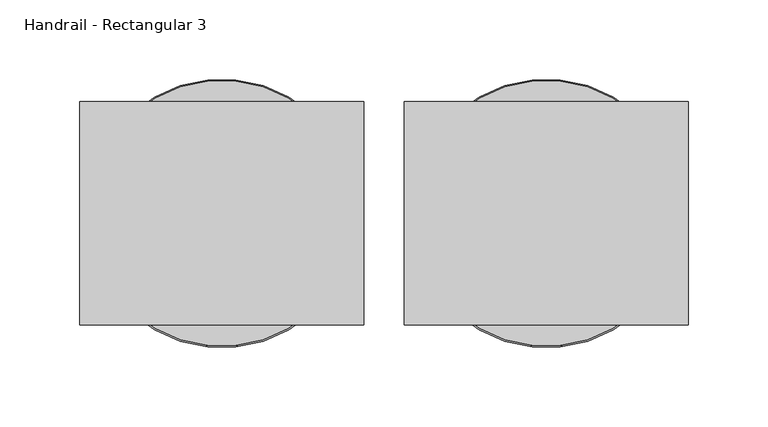
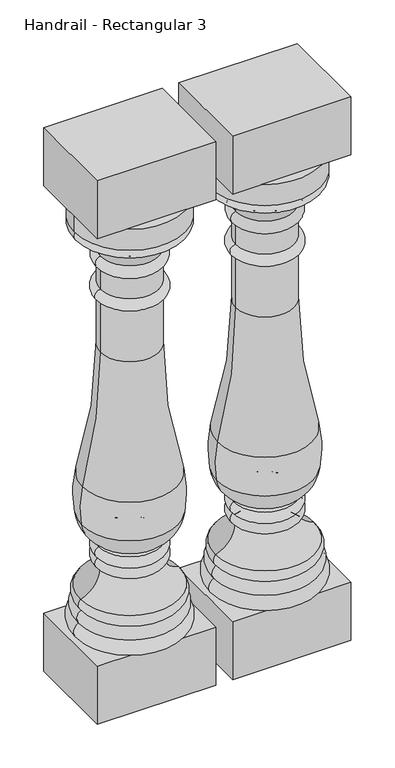
"""IFC4 building model written with IfcOpenShell, lengths in millimetres: railing geometry, Handrail - Rectangular 3."""

from ifc_helpers import new_model, si_unit, point, frame, origin, place, context, project, spatial, polyline, circle_curve, ellipse_curve, trimmed, outline, extrude, source, transform, mapped, element, save
from ifc_brep_helpers import plane_surface, cylinder_surface, revolved_surface, advanced_brep


def handrail_rectangular_3_94038515(model_context):
    return source(origin(), model_context, "Body", "SolidModel", [
        advanced_brep(
        [(12017.1084395, -1665.6164768, 849.3125), (12183.7959395, -1665.6164768, 849.3125), (12183.7959395, -1665.6164768, 882.65), (12017.1084395, -1665.6164768, 882.65), (12020.2834395, -1665.6164768, 849.3125), (12180.6209395, -1665.6164768, 849.3125), (12020.2834395, -1665.6164768, 835.025), (12180.6209395, -1665.6164768, 835.025), (12056.7959395, -1665.6164768, 796.925), (12144.1084395, -1665.6164768, 796.925), (12056.7959395, -1665.6164768, 777.875), (12144.1084395, -1665.6164768, 777.875), (12056.7959395, -1665.6164768, 744.5375), (12144.1084395, -1665.6164768, 744.5375), (12056.7959395, -1665.6164768, 727.075), (12144.1084395, -1665.6164768, 727.075), (12056.7959395, -1665.6164768, 644.525), (12144.1084395, -1665.6164768, 644.525), (12029.6074221, -1665.6164768, 440.2065586), (12171.296957, -1665.6164768, 440.2065586), (12028.4170661, -1665.6164768, 379.6643134), (12172.487313, -1665.6164768, 379.6643134), (12055.6281246, -1665.6164768, 340.8286685), (12145.2762545, -1665.6164768, 340.8286685), (12053.9028429, -1665.6164768, 336.3463085), (12147.0015362, -1665.6164768, 336.3463085), (12052.8271895, -1665.6164768, 319.0875), (12148.0771895, -1665.6164768, 319.0875), (12056.0021895, -1665.6164768, 301.625), (12144.9021895, -1665.6164768, 301.625), (12026.6334395, -1665.6164768, 261.9375), (12174.2709395, -1665.6164768, 261.9375), (12027.4271895, -1665.6164768, 244.475), (12173.4771895, -1665.6164768, 244.475), (12023.4584395, -1665.6164768, 225.425), (12177.4459395, -1665.6164768, 225.425), (12020.2834395, -1665.6164768, 203.2), (12180.6209395, -1665.6164768, 203.2), (12100.4521895, -1665.6164768, 203.2), (12100.4521895, -1665.6164768, 882.65)],
        [
            (0, 1, circle_curve(frame((12100.4521895, -1665.6164768, 849.3125), z_axis=(0.0, 0.0, 1.0), x_axis=(1.0, 0.0, 0.0)), 83.34375)),
            (1, 2),
            (2, 3, circle_curve(frame((12100.4521895, -1665.6164768, 882.65), z_axis=(0.0, 0.0, -1.0), x_axis=(1.0, 0.0, 0.0)), 83.34375)),
            (3, 0),
            (1, 0, circle_curve(frame((12100.4521895, -1665.6164768, 849.3125), z_axis=(0.0, 0.0, 1.0), x_axis=(1.0, 0.0, 0.0)), 83.34375)),
            (3, 2, circle_curve(frame((12100.4521895, -1665.6164768, 882.65), z_axis=(0.0, 0.0, -1.0), x_axis=(1.0, 0.0, 0.0)), 83.34375)),
            (4, 5, circle_curve(frame((12100.4521895, -1665.6164768, 849.3125), z_axis=(0.0, 0.0, 1.0), x_axis=(1.0, 0.0, 0.0)), 80.16875)),
            (5, 1),
            (0, 4),
            (5, 4, circle_curve(frame((12100.4521895, -1665.6164768, 849.3125), z_axis=(0.0, 0.0, 1.0), x_axis=(1.0, 0.0, 0.0)), 80.16875)),
            (6, 7, circle_curve(frame((12100.4521895, -1665.6164768, 835.025), z_axis=(0.0, 0.0, 1.0), x_axis=(1.0, 0.0, 0.0)), 80.16875)),
            (7, 5, circle_curve(frame((12174.1717208, -1665.6164768, 842.16875), z_axis=(0.0, -1.0, 0.0), x_axis=(1.0, 0.0, 0.0)), 9.6242187)),
            (4, 6, circle_curve(frame((12026.7326583, -1665.6164768, 842.16875), z_axis=(0.0, -1.0, 0.0), x_axis=(-1.0, 0.0, 0.0)), 9.6242187)),
            (7, 6, circle_curve(frame((12100.4521895, -1665.6164768, 835.025), z_axis=(0.0, 0.0, 1.0), x_axis=(1.0, 0.0, 0.0)), 80.16875)),
            (8, 9, circle_curve(frame((12100.4521895, -1665.6164768, 796.925), z_axis=(0.0, 0.0, 1.0), x_axis=(1.0, 0.0, 0.0)), 43.65625)),
            (9, 7, circle_curve(frame((12199.525244, -1665.6164768, 780.362802), z_axis=(0.0, 1.0, 0.0), x_axis=(1.0, 0.0, 0.0)), 57.8388159)),
            (6, 8, circle_curve(frame((12001.3791351, -1665.6164768, 780.362802), z_axis=(0.0, 1.0, 0.0), x_axis=(-1.0, 0.0, 0.0)), 57.8388159)),
            (9, 8, circle_curve(frame((12100.4521895, -1665.6164768, 796.925), z_axis=(0.0, 0.0, 1.0), x_axis=(1.0, 0.0, 0.0)), 43.65625)),
            (10, 11, circle_curve(frame((12100.4521895, -1665.6164768, 777.875), z_axis=(0.0, 0.0, 1.0), x_axis=(1.0, 0.0, 0.0)), 43.65625)),
            (11, 9, circle_curve(frame((12142.3621895, -1665.6164768, 787.4), z_axis=(0.0, -1.0, 0.0), x_axis=(1.0, 0.0, 0.0)), 9.68375)),
            (8, 10, circle_curve(frame((12058.5421895, -1665.6164768, 787.4), z_axis=(0.0, -1.0, 0.0), x_axis=(-1.0, 0.0, 0.0)), 9.68375)),
            (11, 10, circle_curve(frame((12100.4521895, -1665.6164768, 777.875), z_axis=(0.0, 0.0, 1.0), x_axis=(1.0, 0.0, 0.0)), 43.65625)),
            (12, 13, circle_curve(frame((12100.4521895, -1665.6164768, 744.5375), z_axis=(0.0, 0.0, 1.0), x_axis=(1.0, 0.0, 0.0)), 43.65625)),
            (13, 11),
            (10, 12),
            (13, 12, circle_curve(frame((12100.4521895, -1665.6164768, 744.5375), z_axis=(0.0, 0.0, 1.0), x_axis=(1.0, 0.0, 0.0)), 43.65625)),
            (14, 15, circle_curve(frame((12100.4521895, -1665.6164768, 727.075), z_axis=(0.0, 0.0, 1.0), x_axis=(1.0, 0.0, 0.0)), 43.65625)),
            (15, 13, circle_curve(frame((12144.1084395, -1665.6164768, 735.80625), z_axis=(0.0, -1.0, 0.0), x_axis=(1.0, 0.0, 0.0)), 8.73125)),
            (12, 14, circle_curve(frame((12056.7959395, -1665.6164768, 735.80625), z_axis=(0.0, -1.0, 0.0), x_axis=(-1.0, 0.0, 0.0)), 8.73125)),
            (15, 14, circle_curve(frame((12100.4521895, -1665.6164768, 727.075), z_axis=(0.0, 0.0, 1.0), x_axis=(1.0, 0.0, 0.0)), 43.65625)),
            (16, 17, circle_curve(frame((12100.4521895, -1665.6164768, 644.525), z_axis=(0.0, 0.0, 1.0), x_axis=(1.0, 0.0, 0.0)), 43.65625)),
            (17, 15),
            (14, 16),
            (17, 16, circle_curve(frame((12100.4521895, -1665.6164768, 644.525), z_axis=(0.0, 0.0, 1.0), x_axis=(1.0, 0.0, 0.0)), 43.65625)),
            (18, 19, circle_curve(frame((12100.4521895, -1665.6164768, 440.2065586), z_axis=(0.0, 0.0, 1.0), x_axis=(1.0, 0.0, 0.0)), 70.8447675)),
            (19, 17, circle_curve(frame((12878.8851891, -1665.6164768, 638.333048), z_axis=(0.0, 1.0, 0.0), x_axis=(1.0, 0.0, 0.0)), 734.8028389)),
            (16, 18, circle_curve(frame((11322.01919, -1665.6164768, 638.333048), z_axis=(0.0, 1.0, 0.0), x_axis=(-1.0, 0.0, 0.0)), 734.8028389)),
            (19, 18, circle_curve(frame((12100.4521895, -1665.6164768, 440.2065586), z_axis=(0.0, 0.0, 1.0), x_axis=(1.0, 0.0, 0.0)), 70.8447675)),
            (20, 21, circle_curve(frame((12100.4521895, -1665.6164768, 379.6643134), z_axis=(0.0, 0.0, 1.0), x_axis=(1.0, 0.0, 0.0)), 72.0351235)),
            (21, 19, circle_curve(frame((12013.3983349, -1665.6164768, 406.819198), z_axis=(0.0, -1.0, 0.0), x_axis=(1.0, 0.0, 0.0)), 161.3898718)),
            (18, 20, circle_curve(frame((12187.5060442, -1665.6164768, 406.819198), z_axis=(0.0, -1.0, 0.0), x_axis=(-1.0, 0.0, 0.0)), 161.3898718)),
            (21, 20, circle_curve(frame((12100.4521895, -1665.6164768, 379.6643134), z_axis=(0.0, 0.0, 1.0), x_axis=(1.0, 0.0, 0.0)), 72.0351235)),
            (22, 23, circle_curve(frame((12100.4521895, -1665.6164768, 340.8286685), z_axis=(0.0, 0.0, 1.0), x_axis=(1.0, 0.0, 0.0)), 44.8240649)),
            (23, 21, circle_curve(frame((12122.7572912, -1665.6164768, 385.5579203), z_axis=(0.0, -1.0, 0.0), x_axis=(1.0, 0.0, 0.0)), 50.0780358)),
            (20, 22, circle_curve(frame((12078.1470879, -1665.6164768, 385.5579203), z_axis=(0.0, -1.0, 0.0), x_axis=(-1.0, 0.0, 0.0)), 50.0780358)),
            (23, 22, circle_curve(frame((12100.4521895, -1665.6164768, 340.8286685), z_axis=(0.0, 0.0, 1.0), x_axis=(1.0, 0.0, 0.0)), 44.8240649)),
            (24, 25, circle_curve(frame((12100.4521895, -1665.6164768, 336.3463085), z_axis=(0.0, 0.0, 1.0), x_axis=(1.0, 0.0, 0.0)), 46.5493467)),
            (25, 23, circle_curve(frame((12148.0771895, -1665.6164768, 339.3335472), z_axis=(0.0, 1.0, 0.0), x_axis=(1.0, 0.0, 0.0)), 3.175)),
            (22, 24, circle_curve(frame((12052.8271895, -1665.6164768, 339.3335472), z_axis=(0.0, 1.0, 0.0), x_axis=(-1.0, 0.0, 0.0)), 3.175)),
            (25, 24, circle_curve(frame((12100.4521895, -1665.6164768, 336.3463085), z_axis=(0.0, 0.0, 1.0), x_axis=(1.0, 0.0, 0.0)), 46.5493467)),
            (26, 27, circle_curve(frame((12100.4521895, -1665.6164768, 319.0875), z_axis=(0.0, 0.0, 1.0), x_axis=(1.0, 0.0, 0.0)), 47.625)),
            (27, 25, circle_curve(frame((12143.0008248, -1665.6164768, 327.4340404), z_axis=(0.0, -1.0, 0.0), x_axis=(1.0, 0.0, 0.0)), 9.7690437)),
            (24, 26, circle_curve(frame((12057.9035543, -1665.6164768, 327.4340404), z_axis=(0.0, -1.0, 0.0), x_axis=(-1.0, 0.0, 0.0)), 9.7690437)),
            (27, 26, circle_curve(frame((12100.4521895, -1665.6164768, 319.0875), z_axis=(0.0, 0.0, 1.0), x_axis=(1.0, 0.0, 0.0)), 47.625)),
            (28, 29, circle_curve(frame((12100.4521895, -1665.6164768, 301.625), z_axis=(0.0, 0.0, 1.0), x_axis=(1.0, 0.0, 0.0)), 44.45)),
            (29, 27, circle_curve(frame((12143.4635177, -1665.6164768, 310.9064631), z_axis=(0.0, -1.0, 0.0), x_axis=(1.0, 0.0, 0.0)), 9.3923018)),
            (26, 28, circle_curve(frame((12057.4408614, -1665.6164768, 310.9064631), z_axis=(0.0, -1.0, 0.0), x_axis=(-1.0, 0.0, 0.0)), 9.3923018)),
            (29, 28, circle_curve(frame((12100.4521895, -1665.6164768, 301.625), z_axis=(0.0, 0.0, 1.0), x_axis=(1.0, 0.0, 0.0)), 44.45)),
            (30, 31, circle_curve(frame((12100.4521895, -1665.6164768, 261.9375), z_axis=(0.0, 0.0, 1.0), x_axis=(1.0, 0.0, 0.0)), 73.81875)),
            (31, 29, circle_curve(frame((12186.4024429, -1665.6164768, 301.625), z_axis=(0.0, 1.0, 0.0), x_axis=(1.0, 0.0, 0.0)), 41.5002534)),
            (28, 30, circle_curve(frame((12014.5019362, -1665.6164768, 301.625), z_axis=(0.0, 1.0, 0.0), x_axis=(-1.0, 0.0, 0.0)), 41.5002534)),
            (31, 30, circle_curve(frame((12100.4521895, -1665.6164768, 261.9375), z_axis=(0.0, 0.0, 1.0), x_axis=(1.0, 0.0, 0.0)), 73.81875)),
            (32, 33, circle_curve(frame((12100.4521895, -1665.6164768, 244.475), z_axis=(0.0, 0.0, 1.0), x_axis=(1.0, 0.0, 0.0)), 73.025)),
            (33, 31, circle_curve(frame((12164.9664257, -1665.6164768, 253.6111427), z_axis=(0.0, -1.0, 0.0), x_axis=(1.0, 0.0, 0.0)), 12.4860804)),
            (30, 32, circle_curve(frame((12035.9379534, -1665.6164768, 253.6111427), z_axis=(0.0, -1.0, 0.0), x_axis=(-1.0, 0.0, 0.0)), 12.4860804)),
            (33, 32, circle_curve(frame((12100.4521895, -1665.6164768, 244.475), z_axis=(0.0, 0.0, 1.0), x_axis=(1.0, 0.0, 0.0)), 73.025)),
            (34, 35, circle_curve(frame((12100.4521895, -1665.6164768, 225.425), z_axis=(0.0, 0.0, 1.0), x_axis=(1.0, 0.0, 0.0)), 76.99375)),
            (35, 33, circle_curve(frame((12166.8024736, -1665.6164768, 233.1460227), z_axis=(0.0, -1.0, 0.0), x_axis=(1.0, 0.0, 0.0)), 13.1490516)),
            (32, 34, circle_curve(frame((12034.1019054, -1665.6164768, 233.1460227), z_axis=(0.0, -1.0, 0.0), x_axis=(-1.0, 0.0, 0.0)), 13.1490516)),
            (35, 34, circle_curve(frame((12100.4521895, -1665.6164768, 225.425), z_axis=(0.0, 0.0, 1.0), x_axis=(1.0, 0.0, 0.0)), 76.99375)),
            (36, 37, circle_curve(frame((12100.4521895, -1665.6164768, 203.2), z_axis=(0.0, 0.0, 1.0), x_axis=(1.0, 0.0, 0.0)), 80.16875)),
            (37, 35, circle_curve(frame((12170.4722788, -1665.6164768, 213.089477), z_axis=(0.0, -1.0, 0.0), x_axis=(1.0, 0.0, 0.0)), 14.1702883)),
            (34, 36, circle_curve(frame((12030.4321003, -1665.6164768, 213.089477), z_axis=(0.0, -1.0, 0.0), x_axis=(-1.0, 0.0, 0.0)), 14.1702883)),
            (37, 36, circle_curve(frame((12100.4521895, -1665.6164768, 203.2), z_axis=(0.0, 0.0, 1.0), x_axis=(1.0, 0.0, 0.0)), 80.16875)),
            (38, 37),
            (36, 38),
            (2, 39),
            (39, 3),
        ],
        [
            cylinder_surface(frame((12100.4521895, -1665.6164768, 831.85), z_axis=(0.0, 0.0, -1.0), x_axis=(1.0, 0.0, 0.0)), 83.34375),
            plane_surface(frame((12100.4521895, -1665.6164768, 849.3125), z_axis=(0.0, 0.0, -1.0), x_axis=(1.0, 0.0, 0.0))),
            revolved_surface(trimmed(ellipse_curve(frame((12174.1717208, -1665.6164768, 842.16875), z_axis=(0.0, 1.0, 0.0), x_axis=(1.0, 0.0, 0.0)), 9.6242187, 9.6242187), [point((12180.6209395, -1665.6164768, 849.3125))], [point((12180.6209395, -1665.6164768, 835.025))], True, "CARTESIAN"), (12100.4521895, -1665.6164768, 831.85), (0.0, 0.0, -1.0)),
            revolved_surface(trimmed(ellipse_curve(frame((12199.525244, -1665.6164768, 780.362802), z_axis=(0.0, -1.0, 0.0), x_axis=(1.0, 0.0, 0.0)), 57.8388159, 57.8388159), [point((12180.6209395, -1665.6164768, 835.025))], [point((12144.1084395, -1665.6164768, 796.925))], True, "CARTESIAN"), (12100.4521895, -1665.6164768, 831.85), (0.0, 0.0, -1.0)),
            revolved_surface(trimmed(ellipse_curve(frame((12142.3621895, -1665.6164768, 787.4), z_axis=(0.0, 1.0, 0.0), x_axis=(1.0, 0.0, 0.0)), 9.68375, 9.68375), [point((12144.1084395, -1665.6164768, 796.925))], [point((12144.1084395, -1665.6164768, 777.875))], True, "CARTESIAN"), (12100.4521895, -1665.6164768, 831.85), (0.0, 0.0, -1.0)),
            cylinder_surface(frame((12100.4521895, -1665.6164768, 831.85), z_axis=(0.0, 0.0, -1.0), x_axis=(1.0, 0.0, 0.0)), 43.65625),
            revolved_surface(trimmed(ellipse_curve(frame((12144.1084395, -1665.6164768, 735.80625), z_axis=(0.0, 1.0, 0.0), x_axis=(1.0, 0.0, 0.0)), 8.73125, 8.73125), [point((12144.1084395, -1665.6164768, 744.5375))], [point((12144.1084395, -1665.6164768, 727.075))], True, "CARTESIAN"), (12100.4521895, -1665.6164768, 831.85), (0.0, 0.0, -1.0)),
            revolved_surface(trimmed(ellipse_curve(frame((12878.8851891, -1665.6164768, 638.333048), z_axis=(0.0, -1.0, 0.0), x_axis=(1.0, 0.0, 0.0)), 734.8028389, 734.8028389), [point((12144.1084395, -1665.6164768, 644.525))], [point((12171.296957, -1665.6164768, 440.2065586))], True, "CARTESIAN"), (12100.4521895, -1665.6164768, 831.85), (0.0, 0.0, -1.0)),
            revolved_surface(trimmed(ellipse_curve(frame((12013.3983349, -1665.6164768, 406.819198), z_axis=(0.0, 1.0, 0.0), x_axis=(1.0, 0.0, 0.0)), 161.3898718, 161.3898718), [point((12171.296957, -1665.6164768, 440.2065586))], [point((12172.487313, -1665.6164768, 379.6643134))], True, "CARTESIAN"), (12100.4521895, -1665.6164768, 831.85), (0.0, 0.0, -1.0)),
            revolved_surface(trimmed(ellipse_curve(frame((12122.7572912, -1665.6164768, 385.5579203), z_axis=(0.0, 1.0, 0.0), x_axis=(1.0, 0.0, 0.0)), 50.0780358, 50.0780358), [point((12172.487313, -1665.6164768, 379.6643134))], [point((12145.2762545, -1665.6164768, 340.8286685))], True, "CARTESIAN"), (12100.4521895, -1665.6164768, 831.85), (0.0, 0.0, -1.0)),
            revolved_surface(trimmed(ellipse_curve(frame((12148.0771895, -1665.6164768, 339.3335472), z_axis=(0.0, -1.0, 0.0), x_axis=(1.0, 0.0, 0.0)), 3.175, 3.175), [point((12145.2762545, -1665.6164768, 340.8286685))], [point((12147.0015362, -1665.6164768, 336.3463085))], True, "CARTESIAN"), (12100.4521895, -1665.6164768, 831.85), (0.0, 0.0, -1.0)),
            revolved_surface(trimmed(ellipse_curve(frame((12143.0008248, -1665.6164768, 327.4340404), z_axis=(0.0, 1.0, 0.0), x_axis=(1.0, 0.0, 0.0)), 9.7690437, 9.7690437), [point((12147.0015362, -1665.6164768, 336.3463085))], [point((12148.0771895, -1665.6164768, 319.0875))], True, "CARTESIAN"), (12100.4521895, -1665.6164768, 831.85), (0.0, 0.0, -1.0)),
            revolved_surface(trimmed(ellipse_curve(frame((12143.4635177, -1665.6164768, 310.9064631), z_axis=(0.0, 1.0, 0.0), x_axis=(1.0, 0.0, 0.0)), 9.3923018, 9.3923018), [point((12148.0771895, -1665.6164768, 319.0875))], [point((12144.9021895, -1665.6164768, 301.625))], True, "CARTESIAN"), (12100.4521895, -1665.6164768, 831.85), (0.0, 0.0, -1.0)),
            revolved_surface(trimmed(ellipse_curve(frame((12186.4024429, -1665.6164768, 301.625), z_axis=(0.0, -1.0, 0.0), x_axis=(1.0, 0.0, 0.0)), 41.5002534, 41.5002534), [point((12144.9021895, -1665.6164768, 301.625))], [point((12174.2709395, -1665.6164768, 261.9375))], True, "CARTESIAN"), (12100.4521895, -1665.6164768, 831.85), (0.0, 0.0, -1.0)),
            revolved_surface(trimmed(ellipse_curve(frame((12164.9664257, -1665.6164768, 253.6111427), z_axis=(0.0, 1.0, 0.0), x_axis=(1.0, 0.0, 0.0)), 12.4860804, 12.4860804), [point((12174.2709395, -1665.6164768, 261.9375))], [point((12173.4771895, -1665.6164768, 244.475))], True, "CARTESIAN"), (12100.4521895, -1665.6164768, 831.85), (0.0, 0.0, -1.0)),
            revolved_surface(trimmed(ellipse_curve(frame((12166.8024736, -1665.6164768, 233.1460227), z_axis=(0.0, 1.0, 0.0), x_axis=(1.0, 0.0, 0.0)), 13.1490516, 13.1490516), [point((12173.4771895, -1665.6164768, 244.475))], [point((12177.4459395, -1665.6164768, 225.425))], True, "CARTESIAN"), (12100.4521895, -1665.6164768, 831.85), (0.0, 0.0, -1.0)),
            revolved_surface(trimmed(ellipse_curve(frame((12170.4722788, -1665.6164768, 213.089477), z_axis=(0.0, 1.0, 0.0), x_axis=(1.0, 0.0, 0.0)), 14.1702883, 14.1702883), [point((12177.4459395, -1665.6164768, 225.425))], [point((12180.6209395, -1665.6164768, 203.2))], True, "CARTESIAN"), (12100.4521895, -1665.6164768, 831.85), (0.0, 0.0, -1.0)),
            plane_surface(frame((12100.4521895, -1665.6164768, 203.2), z_axis=(0.0, 0.0, -1.0), x_axis=(1.0, 0.0, 0.0))),
            plane_surface(frame((12100.4521895, -1665.6164768, 882.65), z_axis=(0.0, 0.0, 1.0), x_axis=(1.0, 0.0, 0.0))),
        ],
        [
            (0, [[1, 2, 3, 4]]),
            (0, [[5, -4, 6, -2]]),
            (1, [[7, 8, -1, 9]]),
            (1, [[10, -9, -5, -8]]),
            (2, [[11, 12, -7, 13]]),
            (2, [[14, -13, -10, -12]]),
            (3, [[15, 16, -11, 17]]),
            (3, [[18, -17, -14, -16]]),
            (4, [[19, 20, -15, 21]]),
            (4, [[22, -21, -18, -20]]),
            (5, [[23, 24, -19, 25]]),
            (5, [[26, -25, -22, -24]]),
            (6, [[27, 28, -23, 29]]),
            (6, [[30, -29, -26, -28]]),
            (5, [[31, 32, -27, 33]]),
            (5, [[34, -33, -30, -32]]),
            (7, [[35, 36, -31, 37]]),
            (7, [[38, -37, -34, -36]]),
            (8, [[39, 40, -35, 41]]),
            (8, [[42, -41, -38, -40]]),
            (9, [[43, 44, -39, 45]]),
            (9, [[46, -45, -42, -44]]),
            (10, [[47, 48, -43, 49]]),
            (10, [[50, -49, -46, -48]]),
            (11, [[51, 52, -47, 53]]),
            (11, [[54, -53, -50, -52]]),
            (12, [[55, 56, -51, 57]]),
            (12, [[58, -57, -54, -56]]),
            (13, [[59, 60, -55, 61]]),
            (13, [[62, -61, -58, -60]]),
            (14, [[63, 64, -59, 65]]),
            (14, [[66, -65, -62, -64]]),
            (15, [[67, 68, -63, 69]]),
            (15, [[70, -69, -66, -68]]),
            (16, [[71, 72, -67, 73]]),
            (16, [[74, -73, -70, -72]]),
            (17, [[75, -71, 76]]),
            (17, [[-76, -74, -75]]),
            (18, [[-3, 77, 78]]),
            (18, [[-6, -78, -77]]),
        ],
    ),
        extrude(outline(polyline([(12011.5521895, -1735.4664768), (12011.5521895, -1595.7664768), (12189.3521895, -1595.7664768), (12189.3521895, -1735.4664768), (12011.5521895, -1735.4664768)])), frame((0.0, 0.0, 111.125), z_axis=(0.0, 0.0, 1.0), x_axis=(1.0, 0.0, 0.0)), (0.0, 0.0, 1.0), 92.075),
        extrude(outline(polyline([(12011.5521895, -1595.7664768), (12189.3521895, -1595.7664768), (12189.3521895, -1735.4664768), (12011.5521895, -1735.4664768), (12011.5521895, -1595.7664768)])), frame((0.0, 0.0, 882.65), z_axis=(0.0, 0.0, 1.0), x_axis=(1.0, 0.0, 0.0)), (0.0, 0.0, 1.0), 92.075),
        advanced_brep(
        [(11813.9084395, -1665.6164768, 849.3125), (11980.5959395, -1665.6164768, 849.3125), (11980.5959395, -1665.6164768, 882.65), (11813.9084395, -1665.6164768, 882.65), (11817.0834395, -1665.6164768, 849.3125), (11977.4209395, -1665.6164768, 849.3125), (11817.0834395, -1665.6164768, 835.025), (11977.4209395, -1665.6164768, 835.025), (11853.5959395, -1665.6164768, 796.925), (11940.9084395, -1665.6164768, 796.925), (11853.5959395, -1665.6164768, 777.875), (11940.9084395, -1665.6164768, 777.875), (11853.5959395, -1665.6164768, 744.5375), (11940.9084395, -1665.6164768, 744.5375), (11853.5959395, -1665.6164768, 727.075), (11940.9084395, -1665.6164768, 727.075), (11853.5959395, -1665.6164768, 644.525), (11940.9084395, -1665.6164768, 644.525), (11826.4074221, -1665.6164768, 440.2065586), (11968.096957, -1665.6164768, 440.2065586), (11825.2170661, -1665.6164768, 379.6643134), (11969.287313, -1665.6164768, 379.6643134), (11852.4281246, -1665.6164768, 340.8286685), (11942.0762545, -1665.6164768, 340.8286685), (11850.7028429, -1665.6164768, 336.3463085), (11943.8015362, -1665.6164768, 336.3463085), (11849.6271895, -1665.6164768, 319.0875), (11944.8771895, -1665.6164768, 319.0875), (11852.8021895, -1665.6164768, 301.625), (11941.7021895, -1665.6164768, 301.625), (11823.4334395, -1665.6164768, 261.9375), (11971.0709395, -1665.6164768, 261.9375), (11824.2271895, -1665.6164768, 244.475), (11970.2771895, -1665.6164768, 244.475), (11820.2584395, -1665.6164768, 225.425), (11974.2459395, -1665.6164768, 225.425), (11817.0834395, -1665.6164768, 203.2), (11977.4209395, -1665.6164768, 203.2), (11897.2521895, -1665.6164768, 203.2), (11897.2521895, -1665.6164768, 882.65)],
        [
            (0, 1, circle_curve(frame((11897.2521895, -1665.6164768, 849.3125), z_axis=(0.0, 0.0, 1.0), x_axis=(1.0, 0.0, 0.0)), 83.34375)),
            (1, 2),
            (2, 3, circle_curve(frame((11897.2521895, -1665.6164768, 882.65), z_axis=(0.0, 0.0, -1.0), x_axis=(1.0, 0.0, 0.0)), 83.34375)),
            (3, 0),
            (1, 0, circle_curve(frame((11897.2521895, -1665.6164768, 849.3125), z_axis=(0.0, 0.0, 1.0), x_axis=(1.0, 0.0, 0.0)), 83.34375)),
            (3, 2, circle_curve(frame((11897.2521895, -1665.6164768, 882.65), z_axis=(0.0, 0.0, -1.0), x_axis=(1.0, 0.0, 0.0)), 83.34375)),
            (4, 5, circle_curve(frame((11897.2521895, -1665.6164768, 849.3125), z_axis=(0.0, 0.0, 1.0), x_axis=(1.0, 0.0, 0.0)), 80.16875)),
            (5, 1),
            (0, 4),
            (5, 4, circle_curve(frame((11897.2521895, -1665.6164768, 849.3125), z_axis=(0.0, 0.0, 1.0), x_axis=(1.0, 0.0, 0.0)), 80.16875)),
            (6, 7, circle_curve(frame((11897.2521895, -1665.6164768, 835.025), z_axis=(0.0, 0.0, 1.0), x_axis=(1.0, 0.0, 0.0)), 80.16875)),
            (7, 5, circle_curve(frame((11970.9717208, -1665.6164768, 842.16875), z_axis=(0.0, -1.0, 0.0), x_axis=(1.0, 0.0, 0.0)), 9.6242187)),
            (4, 6, circle_curve(frame((11823.5326583, -1665.6164768, 842.16875), z_axis=(0.0, -1.0, 0.0), x_axis=(-1.0, 0.0, 0.0)), 9.6242187)),
            (7, 6, circle_curve(frame((11897.2521895, -1665.6164768, 835.025), z_axis=(0.0, 0.0, 1.0), x_axis=(1.0, 0.0, 0.0)), 80.16875)),
            (8, 9, circle_curve(frame((11897.2521895, -1665.6164768, 796.925), z_axis=(0.0, 0.0, 1.0), x_axis=(1.0, 0.0, 0.0)), 43.65625)),
            (9, 7, circle_curve(frame((11996.325244, -1665.6164768, 780.362802), z_axis=(0.0, 1.0, 0.0), x_axis=(1.0, 0.0, 0.0)), 57.8388159)),
            (6, 8, circle_curve(frame((11798.1791351, -1665.6164768, 780.362802), z_axis=(0.0, 1.0, 0.0), x_axis=(-1.0, 0.0, 0.0)), 57.8388159)),
            (9, 8, circle_curve(frame((11897.2521895, -1665.6164768, 796.925), z_axis=(0.0, 0.0, 1.0), x_axis=(1.0, 0.0, 0.0)), 43.65625)),
            (10, 11, circle_curve(frame((11897.2521895, -1665.6164768, 777.875), z_axis=(0.0, 0.0, 1.0), x_axis=(1.0, 0.0, 0.0)), 43.65625)),
            (11, 9, circle_curve(frame((11939.1621895, -1665.6164768, 787.4), z_axis=(0.0, -1.0, 0.0), x_axis=(1.0, 0.0, 0.0)), 9.68375)),
            (8, 10, circle_curve(frame((11855.3421895, -1665.6164768, 787.4), z_axis=(0.0, -1.0, 0.0), x_axis=(-1.0, 0.0, 0.0)), 9.68375)),
            (11, 10, circle_curve(frame((11897.2521895, -1665.6164768, 777.875), z_axis=(0.0, 0.0, 1.0), x_axis=(1.0, 0.0, 0.0)), 43.65625)),
            (12, 13, circle_curve(frame((11897.2521895, -1665.6164768, 744.5375), z_axis=(0.0, 0.0, 1.0), x_axis=(1.0, 0.0, 0.0)), 43.65625)),
            (13, 11),
            (10, 12),
            (13, 12, circle_curve(frame((11897.2521895, -1665.6164768, 744.5375), z_axis=(0.0, 0.0, 1.0), x_axis=(1.0, 0.0, 0.0)), 43.65625)),
            (14, 15, circle_curve(frame((11897.2521895, -1665.6164768, 727.075), z_axis=(0.0, 0.0, 1.0), x_axis=(1.0, 0.0, 0.0)), 43.65625)),
            (15, 13, circle_curve(frame((11940.9084395, -1665.6164768, 735.80625), z_axis=(0.0, -1.0, 0.0), x_axis=(1.0, 0.0, 0.0)), 8.73125)),
            (12, 14, circle_curve(frame((11853.5959395, -1665.6164768, 735.80625), z_axis=(0.0, -1.0, 0.0), x_axis=(-1.0, 0.0, 0.0)), 8.73125)),
            (15, 14, circle_curve(frame((11897.2521895, -1665.6164768, 727.075), z_axis=(0.0, 0.0, 1.0), x_axis=(1.0, 0.0, 0.0)), 43.65625)),
            (16, 17, circle_curve(frame((11897.2521895, -1665.6164768, 644.525), z_axis=(0.0, 0.0, 1.0), x_axis=(1.0, 0.0, 0.0)), 43.65625)),
            (17, 15),
            (14, 16),
            (17, 16, circle_curve(frame((11897.2521895, -1665.6164768, 644.525), z_axis=(0.0, 0.0, 1.0), x_axis=(1.0, 0.0, 0.0)), 43.65625)),
            (18, 19, circle_curve(frame((11897.2521895, -1665.6164768, 440.2065586), z_axis=(0.0, 0.0, 1.0), x_axis=(1.0, 0.0, 0.0)), 70.8447675)),
            (19, 17, circle_curve(frame((12675.6851891, -1665.6164768, 638.333048), z_axis=(0.0, 1.0, 0.0), x_axis=(1.0, 0.0, 0.0)), 734.8028389)),
            (16, 18, circle_curve(frame((11118.81919, -1665.6164768, 638.333048), z_axis=(0.0, 1.0, 0.0), x_axis=(-1.0, 0.0, 0.0)), 734.8028389)),
            (19, 18, circle_curve(frame((11897.2521895, -1665.6164768, 440.2065586), z_axis=(0.0, 0.0, 1.0), x_axis=(1.0, 0.0, 0.0)), 70.8447675)),
            (20, 21, circle_curve(frame((11897.2521895, -1665.6164768, 379.6643134), z_axis=(0.0, 0.0, 1.0), x_axis=(1.0, 0.0, 0.0)), 72.0351235)),
            (21, 19, circle_curve(frame((11810.1983349, -1665.6164768, 406.819198), z_axis=(0.0, -1.0, 0.0), x_axis=(1.0, 0.0, 0.0)), 161.3898718)),
            (18, 20, circle_curve(frame((11984.3060442, -1665.6164768, 406.819198), z_axis=(0.0, -1.0, 0.0), x_axis=(-1.0, 0.0, 0.0)), 161.3898718)),
            (21, 20, circle_curve(frame((11897.2521895, -1665.6164768, 379.6643134), z_axis=(0.0, 0.0, 1.0), x_axis=(1.0, 0.0, 0.0)), 72.0351235)),
            (22, 23, circle_curve(frame((11897.2521895, -1665.6164768, 340.8286685), z_axis=(0.0, 0.0, 1.0), x_axis=(1.0, 0.0, 0.0)), 44.8240649)),
            (23, 21, circle_curve(frame((11919.5572912, -1665.6164768, 385.5579203), z_axis=(0.0, -1.0, 0.0), x_axis=(1.0, 0.0, 0.0)), 50.0780358)),
            (20, 22, circle_curve(frame((11874.9470879, -1665.6164768, 385.5579203), z_axis=(0.0, -1.0, 0.0), x_axis=(-1.0, 0.0, 0.0)), 50.0780358)),
            (23, 22, circle_curve(frame((11897.2521895, -1665.6164768, 340.8286685), z_axis=(0.0, 0.0, 1.0), x_axis=(1.0, 0.0, 0.0)), 44.8240649)),
            (24, 25, circle_curve(frame((11897.2521895, -1665.6164768, 336.3463085), z_axis=(0.0, 0.0, 1.0), x_axis=(1.0, 0.0, 0.0)), 46.5493467)),
            (25, 23, circle_curve(frame((11944.8771895, -1665.6164768, 339.3335472), z_axis=(0.0, 1.0, 0.0), x_axis=(1.0, 0.0, 0.0)), 3.175)),
            (22, 24, circle_curve(frame((11849.6271895, -1665.6164768, 339.3335472), z_axis=(0.0, 1.0, 0.0), x_axis=(-1.0, 0.0, 0.0)), 3.175)),
            (25, 24, circle_curve(frame((11897.2521895, -1665.6164768, 336.3463085), z_axis=(0.0, 0.0, 1.0), x_axis=(1.0, 0.0, 0.0)), 46.5493467)),
            (26, 27, circle_curve(frame((11897.2521895, -1665.6164768, 319.0875), z_axis=(0.0, 0.0, 1.0), x_axis=(1.0, 0.0, 0.0)), 47.625)),
            (27, 25, circle_curve(frame((11939.8008248, -1665.6164768, 327.4340404), z_axis=(0.0, -1.0, 0.0), x_axis=(1.0, 0.0, 0.0)), 9.7690437)),
            (24, 26, circle_curve(frame((11854.7035543, -1665.6164768, 327.4340404), z_axis=(0.0, -1.0, 0.0), x_axis=(-1.0, 0.0, 0.0)), 9.7690437)),
            (27, 26, circle_curve(frame((11897.2521895, -1665.6164768, 319.0875), z_axis=(0.0, 0.0, 1.0), x_axis=(1.0, 0.0, 0.0)), 47.625)),
            (28, 29, circle_curve(frame((11897.2521895, -1665.6164768, 301.625), z_axis=(0.0, 0.0, 1.0), x_axis=(1.0, 0.0, 0.0)), 44.45)),
            (29, 27, circle_curve(frame((11940.2635177, -1665.6164768, 310.9064631), z_axis=(0.0, -1.0, 0.0), x_axis=(1.0, 0.0, 0.0)), 9.3923018)),
            (26, 28, circle_curve(frame((11854.2408614, -1665.6164768, 310.9064631), z_axis=(0.0, -1.0, 0.0), x_axis=(-1.0, 0.0, 0.0)), 9.3923018)),
            (29, 28, circle_curve(frame((11897.2521895, -1665.6164768, 301.625), z_axis=(0.0, 0.0, 1.0), x_axis=(1.0, 0.0, 0.0)), 44.45)),
            (30, 31, circle_curve(frame((11897.2521895, -1665.6164768, 261.9375), z_axis=(0.0, 0.0, 1.0), x_axis=(1.0, 0.0, 0.0)), 73.81875)),
            (31, 29, circle_curve(frame((11983.2024429, -1665.6164768, 301.625), z_axis=(0.0, 1.0, 0.0), x_axis=(1.0, 0.0, 0.0)), 41.5002534)),
            (28, 30, circle_curve(frame((11811.3019362, -1665.6164768, 301.625), z_axis=(0.0, 1.0, 0.0), x_axis=(-1.0, 0.0, 0.0)), 41.5002534)),
            (31, 30, circle_curve(frame((11897.2521895, -1665.6164768, 261.9375), z_axis=(0.0, 0.0, 1.0), x_axis=(1.0, 0.0, 0.0)), 73.81875)),
            (32, 33, circle_curve(frame((11897.2521895, -1665.6164768, 244.475), z_axis=(0.0, 0.0, 1.0), x_axis=(1.0, 0.0, 0.0)), 73.025)),
            (33, 31, circle_curve(frame((11961.7664257, -1665.6164768, 253.6111427), z_axis=(0.0, -1.0, 0.0), x_axis=(1.0, 0.0, 0.0)), 12.4860804)),
            (30, 32, circle_curve(frame((11832.7379534, -1665.6164768, 253.6111427), z_axis=(0.0, -1.0, 0.0), x_axis=(-1.0, 0.0, 0.0)), 12.4860804)),
            (33, 32, circle_curve(frame((11897.2521895, -1665.6164768, 244.475), z_axis=(0.0, 0.0, 1.0), x_axis=(1.0, 0.0, 0.0)), 73.025)),
            (34, 35, circle_curve(frame((11897.2521895, -1665.6164768, 225.425), z_axis=(0.0, 0.0, 1.0), x_axis=(1.0, 0.0, 0.0)), 76.99375)),
            (35, 33, circle_curve(frame((11963.6024736, -1665.6164768, 233.1460227), z_axis=(0.0, -1.0, 0.0), x_axis=(1.0, 0.0, 0.0)), 13.1490516)),
            (32, 34, circle_curve(frame((11830.9019054, -1665.6164768, 233.1460227), z_axis=(0.0, -1.0, 0.0), x_axis=(-1.0, 0.0, 0.0)), 13.1490516)),
            (35, 34, circle_curve(frame((11897.2521895, -1665.6164768, 225.425), z_axis=(0.0, 0.0, 1.0), x_axis=(1.0, 0.0, 0.0)), 76.99375)),
            (36, 37, circle_curve(frame((11897.2521895, -1665.6164768, 203.2), z_axis=(0.0, 0.0, 1.0), x_axis=(1.0, 0.0, 0.0)), 80.16875)),
            (37, 35, circle_curve(frame((11967.2722788, -1665.6164768, 213.089477), z_axis=(0.0, -1.0, 0.0), x_axis=(1.0, 0.0, 0.0)), 14.1702883)),
            (34, 36, circle_curve(frame((11827.2321003, -1665.6164768, 213.089477), z_axis=(0.0, -1.0, 0.0), x_axis=(-1.0, 0.0, 0.0)), 14.1702883)),
            (37, 36, circle_curve(frame((11897.2521895, -1665.6164768, 203.2), z_axis=(0.0, 0.0, 1.0), x_axis=(1.0, 0.0, 0.0)), 80.16875)),
            (38, 37),
            (36, 38),
            (2, 39),
            (39, 3),
        ],
        [
            cylinder_surface(frame((11897.2521895, -1665.6164768, 831.85), z_axis=(0.0, 0.0, -1.0), x_axis=(1.0, 0.0, 0.0)), 83.34375),
            plane_surface(frame((11897.2521895, -1665.6164768, 849.3125), z_axis=(0.0, 0.0, -1.0), x_axis=(1.0, 0.0, 0.0))),
            revolved_surface(trimmed(ellipse_curve(frame((11970.9717208, -1665.6164768, 842.16875), z_axis=(0.0, 1.0, 0.0), x_axis=(1.0, 0.0, 0.0)), 9.6242187, 9.6242187), [point((11977.4209395, -1665.6164768, 849.3125))], [point((11977.4209395, -1665.6164768, 835.025))], True, "CARTESIAN"), (11897.2521895, -1665.6164768, 831.85), (0.0, 0.0, -1.0)),
            revolved_surface(trimmed(ellipse_curve(frame((11996.325244, -1665.6164768, 780.362802), z_axis=(0.0, -1.0, 0.0), x_axis=(1.0, 0.0, 0.0)), 57.8388159, 57.8388159), [point((11977.4209395, -1665.6164768, 835.025))], [point((11940.9084395, -1665.6164768, 796.925))], True, "CARTESIAN"), (11897.2521895, -1665.6164768, 831.85), (0.0, 0.0, -1.0)),
            revolved_surface(trimmed(ellipse_curve(frame((11939.1621895, -1665.6164768, 787.4), z_axis=(0.0, 1.0, 0.0), x_axis=(1.0, 0.0, 0.0)), 9.68375, 9.68375), [point((11940.9084395, -1665.6164768, 796.925))], [point((11940.9084395, -1665.6164768, 777.875))], True, "CARTESIAN"), (11897.2521895, -1665.6164768, 831.85), (0.0, 0.0, -1.0)),
            cylinder_surface(frame((11897.2521895, -1665.6164768, 831.85), z_axis=(0.0, 0.0, -1.0), x_axis=(1.0, 0.0, 0.0)), 43.65625),
            revolved_surface(trimmed(ellipse_curve(frame((11940.9084395, -1665.6164768, 735.80625), z_axis=(0.0, 1.0, 0.0), x_axis=(1.0, 0.0, 0.0)), 8.73125, 8.73125), [point((11940.9084395, -1665.6164768, 744.5375))], [point((11940.9084395, -1665.6164768, 727.075))], True, "CARTESIAN"), (11897.2521895, -1665.6164768, 831.85), (0.0, 0.0, -1.0)),
            revolved_surface(trimmed(ellipse_curve(frame((12675.6851891, -1665.6164768, 638.333048), z_axis=(0.0, -1.0, 0.0), x_axis=(1.0, 0.0, 0.0)), 734.8028389, 734.8028389), [point((11940.9084395, -1665.6164768, 644.525))], [point((11968.096957, -1665.6164768, 440.2065586))], True, "CARTESIAN"), (11897.2521895, -1665.6164768, 831.85), (0.0, 0.0, -1.0)),
            revolved_surface(trimmed(ellipse_curve(frame((11810.1983349, -1665.6164768, 406.819198), z_axis=(0.0, 1.0, 0.0), x_axis=(1.0, 0.0, 0.0)), 161.3898718, 161.3898718), [point((11968.096957, -1665.6164768, 440.2065586))], [point((11969.287313, -1665.6164768, 379.6643134))], True, "CARTESIAN"), (11897.2521895, -1665.6164768, 831.85), (0.0, 0.0, -1.0)),
            revolved_surface(trimmed(ellipse_curve(frame((11919.5572912, -1665.6164768, 385.5579203), z_axis=(0.0, 1.0, 0.0), x_axis=(1.0, 0.0, 0.0)), 50.0780358, 50.0780358), [point((11969.287313, -1665.6164768, 379.6643134))], [point((11942.0762545, -1665.6164768, 340.8286685))], True, "CARTESIAN"), (11897.2521895, -1665.6164768, 831.85), (0.0, 0.0, -1.0)),
            revolved_surface(trimmed(ellipse_curve(frame((11944.8771895, -1665.6164768, 339.3335472), z_axis=(0.0, -1.0, 0.0), x_axis=(1.0, 0.0, 0.0)), 3.175, 3.175), [point((11942.0762545, -1665.6164768, 340.8286685))], [point((11943.8015362, -1665.6164768, 336.3463085))], True, "CARTESIAN"), (11897.2521895, -1665.6164768, 831.85), (0.0, 0.0, -1.0)),
            revolved_surface(trimmed(ellipse_curve(frame((11939.8008248, -1665.6164768, 327.4340404), z_axis=(0.0, 1.0, 0.0), x_axis=(1.0, 0.0, 0.0)), 9.7690437, 9.7690437), [point((11943.8015362, -1665.6164768, 336.3463085))], [point((11944.8771895, -1665.6164768, 319.0875))], True, "CARTESIAN"), (11897.2521895, -1665.6164768, 831.85), (0.0, 0.0, -1.0)),
            revolved_surface(trimmed(ellipse_curve(frame((11940.2635177, -1665.6164768, 310.9064631), z_axis=(0.0, 1.0, 0.0), x_axis=(1.0, 0.0, 0.0)), 9.3923018, 9.3923018), [point((11944.8771895, -1665.6164768, 319.0875))], [point((11941.7021895, -1665.6164768, 301.625))], True, "CARTESIAN"), (11897.2521895, -1665.6164768, 831.85), (0.0, 0.0, -1.0)),
            revolved_surface(trimmed(ellipse_curve(frame((11983.2024429, -1665.6164768, 301.625), z_axis=(0.0, -1.0, 0.0), x_axis=(1.0, 0.0, 0.0)), 41.5002534, 41.5002534), [point((11941.7021895, -1665.6164768, 301.625))], [point((11971.0709395, -1665.6164768, 261.9375))], True, "CARTESIAN"), (11897.2521895, -1665.6164768, 831.85), (0.0, 0.0, -1.0)),
            revolved_surface(trimmed(ellipse_curve(frame((11961.7664257, -1665.6164768, 253.6111427), z_axis=(0.0, 1.0, 0.0), x_axis=(1.0, 0.0, 0.0)), 12.4860804, 12.4860804), [point((11971.0709395, -1665.6164768, 261.9375))], [point((11970.2771895, -1665.6164768, 244.475))], True, "CARTESIAN"), (11897.2521895, -1665.6164768, 831.85), (0.0, 0.0, -1.0)),
            revolved_surface(trimmed(ellipse_curve(frame((11963.6024736, -1665.6164768, 233.1460227), z_axis=(0.0, 1.0, 0.0), x_axis=(1.0, 0.0, 0.0)), 13.1490516, 13.1490516), [point((11970.2771895, -1665.6164768, 244.475))], [point((11974.2459395, -1665.6164768, 225.425))], True, "CARTESIAN"), (11897.2521895, -1665.6164768, 831.85), (0.0, 0.0, -1.0)),
            revolved_surface(trimmed(ellipse_curve(frame((11967.2722788, -1665.6164768, 213.089477), z_axis=(0.0, 1.0, 0.0), x_axis=(1.0, 0.0, 0.0)), 14.1702883, 14.1702883), [point((11974.2459395, -1665.6164768, 225.425))], [point((11977.4209395, -1665.6164768, 203.2))], True, "CARTESIAN"), (11897.2521895, -1665.6164768, 831.85), (0.0, 0.0, -1.0)),
            plane_surface(frame((11897.2521895, -1665.6164768, 203.2), z_axis=(0.0, 0.0, -1.0), x_axis=(1.0, 0.0, 0.0))),
            plane_surface(frame((11897.2521895, -1665.6164768, 882.65), z_axis=(0.0, 0.0, 1.0), x_axis=(1.0, 0.0, 0.0))),
        ],
        [
            (0, [[1, 2, 3, 4]]),
            (0, [[5, -4, 6, -2]]),
            (1, [[7, 8, -1, 9]]),
            (1, [[10, -9, -5, -8]]),
            (2, [[11, 12, -7, 13]]),
            (2, [[14, -13, -10, -12]]),
            (3, [[15, 16, -11, 17]]),
            (3, [[18, -17, -14, -16]]),
            (4, [[19, 20, -15, 21]]),
            (4, [[22, -21, -18, -20]]),
            (5, [[23, 24, -19, 25]]),
            (5, [[26, -25, -22, -24]]),
            (6, [[27, 28, -23, 29]]),
            (6, [[30, -29, -26, -28]]),
            (5, [[31, 32, -27, 33]]),
            (5, [[34, -33, -30, -32]]),
            (7, [[35, 36, -31, 37]]),
            (7, [[38, -37, -34, -36]]),
            (8, [[39, 40, -35, 41]]),
            (8, [[42, -41, -38, -40]]),
            (9, [[43, 44, -39, 45]]),
            (9, [[46, -45, -42, -44]]),
            (10, [[47, 48, -43, 49]]),
            (10, [[50, -49, -46, -48]]),
            (11, [[51, 52, -47, 53]]),
            (11, [[54, -53, -50, -52]]),
            (12, [[55, 56, -51, 57]]),
            (12, [[58, -57, -54, -56]]),
            (13, [[59, 60, -55, 61]]),
            (13, [[62, -61, -58, -60]]),
            (14, [[63, 64, -59, 65]]),
            (14, [[66, -65, -62, -64]]),
            (15, [[67, 68, -63, 69]]),
            (15, [[70, -69, -66, -68]]),
            (16, [[71, 72, -67, 73]]),
            (16, [[74, -73, -70, -72]]),
            (17, [[75, -71, 76]]),
            (17, [[-76, -74, -75]]),
            (18, [[-3, 77, 78]]),
            (18, [[-6, -78, -77]]),
        ],
    ),
        extrude(outline(polyline([(11808.3521895, -1735.4664768), (11808.3521895, -1595.7664768), (11986.1521895, -1595.7664768), (11986.1521895, -1735.4664768), (11808.3521895, -1735.4664768)])), frame((0.0, 0.0, 111.125), z_axis=(0.0, 0.0, 1.0), x_axis=(1.0, 0.0, 0.0)), (0.0, 0.0, 1.0), 92.075),
        extrude(outline(polyline([(11808.3521895, -1595.7664768), (11986.1521895, -1595.7664768), (11986.1521895, -1735.4664768), (11808.3521895, -1735.4664768), (11808.3521895, -1595.7664768)])), frame((0.0, 0.0, 882.65), z_axis=(0.0, 0.0, 1.0), x_axis=(1.0, 0.0, 0.0)), (0.0, 0.0, 1.0), 92.075),
    ])


if __name__ == "__main__":
    model = new_model("IFC4")
    model_context = context("Model", 3, world=origin())
    ifc_project = project(units=[si_unit("LENGTHUNIT", "METRE", prefix="MILLI")], contexts=[model_context])
    site = spatial("IfcSite", under=ifc_project)
    building = spatial("IfcBuilding", under=site)
    placement = place(None, origin())
    handrail_rectangular_3_shape = handrail_rectangular_3_94038515(model_context)
    element("IfcRailing", 1, ObjectType="Handrail - Rectangular 3", at=placement, inside=building, context=model_context, shape_type="MappedRepresentation", body=[
        mapped(handrail_rectangular_3_shape, transform((0.0, 0.0, 0.0), x_axis=(1.0, 0.0, 0.0), y_axis=(0.0, 1.0, 0.0), z_axis=(0.0, 0.0, 1.0))),
    ])
    save(model, "model.ifc")
